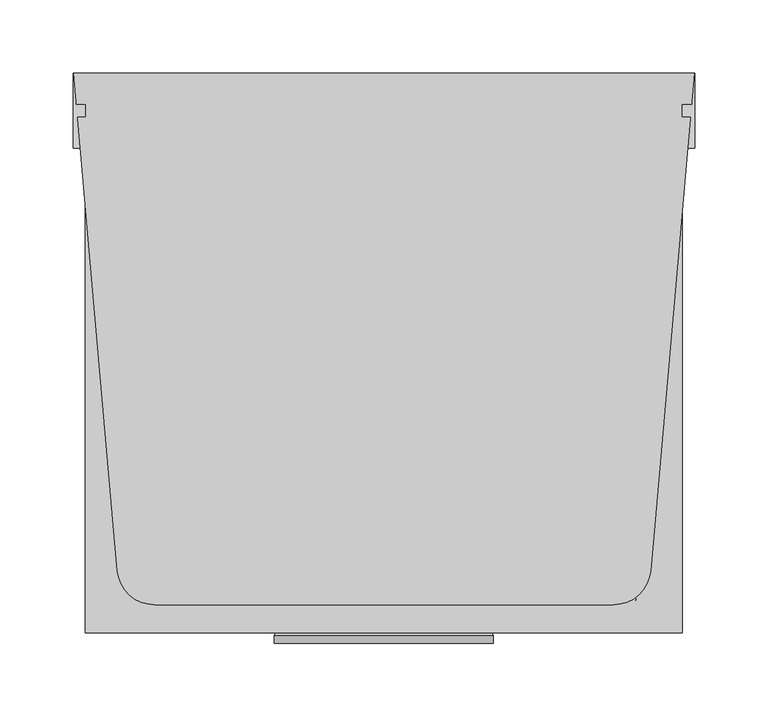
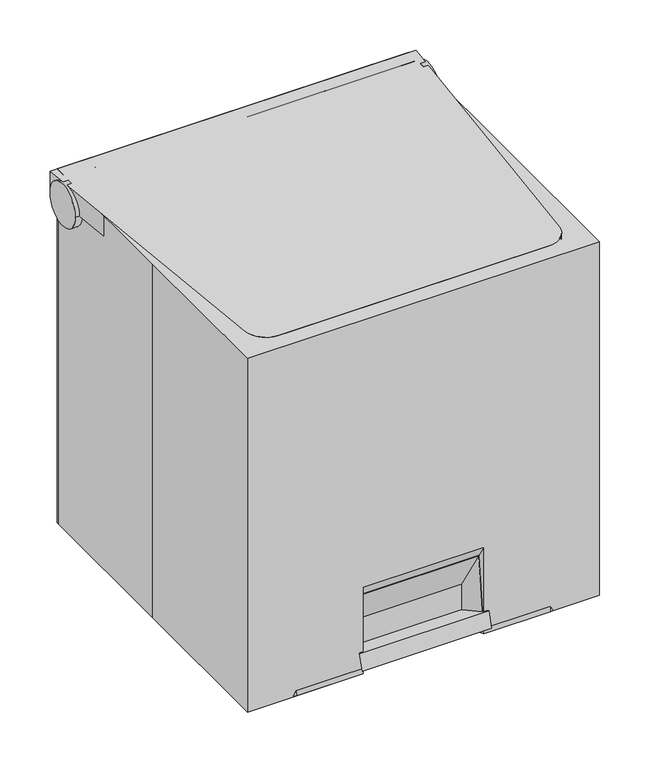
"""IFC4 building model written with IfcOpenShell, lengths in millimetres: proxy geometry, M3073 - Basket, Infectious Waste, Step-On : M0013 - Basket, Infectious Waste, Step-On."""

import ifcopenshell
import ifcopenshell.guid

model = None  # the IFC model being written
_history = None  # IfcOwnerHistory: only IFC2X3 demands one
_inside = {}  # id of a spatial element -> (the spatial element, [elements in it])
_under = {}  # id of a project, library or spatial element -> (it, [spatial elements below it])
_declared = {}  # id of a project -> (the project, [libraries it declares])
_typed = {}  # id of a type object -> (the type object, [elements of that type])
_made_of = {}  # id of a material, layer set ... -> (it, [elements and type objects made of it])


def new_model(schema):
    """Start an empty IFC model of exactly this schema.

    Asked for "IFC4X3", IfcOpenShell would pick the latest addendum, in which some entities
    have other attributes; the version numbers below select the first issue.
    IFC2X3 requires an IfcOwnerHistory on every rooted entity: one is made here for all.
    """
    global model, _history
    if schema == "IFC4X3":
        model = ifcopenshell.file(schema_version=(4, 3, 0, 0))
    else:
        model = ifcopenshell.file(schema=schema)
    _inside.clear()
    _under.clear()
    _declared.clear()
    _typed.clear()
    _made_of.clear()
    _history = None
    if model.schema == "IFC2X3":
        org = make("IfcOrganization", Name="unknown")
        user = make(
            "IfcPersonAndOrganization",
            ThePerson=make("IfcPerson", FamilyName="unknown"),
            TheOrganization=org,
        )
        app = make(
            "IfcApplication",
            ApplicationDeveloper=org,
            Version="unknown",
            ApplicationFullName="unknown",
            ApplicationIdentifier="unknown",
        )
        _history = make(
            "IfcOwnerHistory",
            OwningUser=user,
            OwningApplication=app,
            ChangeAction="ADDED",
            CreationDate=0,
        )
    return model


def make(cls, **values):
    """One entity of the class cls with the attributes given. An attribute that is None is left unset."""
    return model.create_entity(
        cls, **{name: value for name, value in values.items() if value is not None}
    )


def rooted(cls, **values):
    """An entity with a GlobalId (a new one), such as an element, a storey or a relation."""
    return make(cls, GlobalId=ifcopenshell.guid.new(), OwnerHistory=_history, **values)


def si_unit(unit_type, name, prefix=None):
    """IfcSIUnit, for example si_unit("LENGTHUNIT", "METRE", prefix="MILLI")."""
    return make("IfcSIUnit", UnitType=unit_type, Prefix=prefix, Name=name)


def assignment(units):
    """IfcUnitAssignment: the units of a project."""
    return None if units is None else make("IfcUnitAssignment", Units=units)


def point(xyz):
    """IfcCartesianPoint."""
    return None if xyz is None else make("IfcCartesianPoint", Coordinates=xyz)


def direction(xyz):
    """IfcDirection."""
    return None if xyz is None else make("IfcDirection", DirectionRatios=xyz)


def frame(location, z_axis=None, x_axis=None):
    """IfcAxis2Placement3D, a coordinate frame: its origin and axes. An axis left out is left unset."""
    return make(
        "IfcAxis2Placement3D",
        Location=point(location),
        Axis=direction(z_axis),
        RefDirection=direction(x_axis),
    )


def frame_2d(location, x_axis=None):
    """IfcAxis2Placement2D, a coordinate frame in the plane: its origin and x axis."""
    return make(
        "IfcAxis2Placement2D", Location=point(location), RefDirection=direction(x_axis)
    )


def origin():
    """The frame at (0, 0, 0) with its axes left unset."""
    return frame((0.0, 0.0, 0.0))


def place(relative_to, where):
    """IfcLocalPlacement: puts the frame where relative to a parent placement (None: the world)."""
    return make(
        "IfcLocalPlacement", PlacementRelTo=relative_to, RelativePlacement=where
    )


def context(
    kind, dimensions, precision=None, world=None, true_north=None, identifier=None
):
    """IfcGeometricRepresentationContext, for example the 3D "Model" context."""
    return make(
        "IfcGeometricRepresentationContext",
        ContextIdentifier=identifier,
        ContextType=kind,
        CoordinateSpaceDimension=dimensions,
        Precision=precision,
        WorldCoordinateSystem=world,
        TrueNorth=true_north,
    )


def project(units=None, contexts=None):
    """IfcProject with its units and contexts."""
    return rooted(
        "IfcProject",
        Name="project",
        RepresentationContexts=contexts,
        UnitsInContext=assignment(units),
    )


def spatial(cls, under=None, at=None, **own):
    """A site, building, storey or space (cls), placed at a placement, below another one or the project."""
    s = rooted(cls, ObjectPlacement=at, **own)
    if under is not None:
        _under.setdefault(under.id(), (under, []))[1].append(s)
    return s


def polyline(points):
    """IfcPolyline through the points."""
    return make("IfcPolyline", Points=[point(p) for p in points])


def circle_curve(where, radius):
    """IfcCircle in the frame where."""
    return make("IfcCircle", Position=where, Radius=radius)


def ellipse_curve(where, semi_axis1, semi_axis2):
    """IfcEllipse in the frame where."""
    return make(
        "IfcEllipse", Position=where, SemiAxis1=semi_axis1, SemiAxis2=semi_axis2
    )


def trimmed(basis, trim1, trim2, sense, master):
    """IfcTrimmedCurve: the piece of a basis curve between two trims."""
    return make(
        "IfcTrimmedCurve",
        BasisCurve=basis,
        Trim1=trim1,
        Trim2=trim2,
        SenseAgreement=sense,
        MasterRepresentation=master,
    )


def segment(curve, same_sense, transition):
    """IfcCompositeCurveSegment."""
    return make(
        "IfcCompositeCurveSegment",
        Transition=transition,
        SameSense=same_sense,
        ParentCurve=curve,
    )


def composite_curve(segments, self_intersect=None):
    """IfcCompositeCurve: segments joined end to end."""
    return make("IfcCompositeCurve", Segments=segments, SelfIntersect=self_intersect)


def outline(outer, holes=None, kind="AREA"):
    """IfcArbitraryClosedProfileDef: a profile drawn as a closed curve; with holes, ...WithVoids."""
    if holes is None:
        return make("IfcArbitraryClosedProfileDef", ProfileType=kind, OuterCurve=outer)
    return make(
        "IfcArbitraryProfileDefWithVoids",
        ProfileType=kind,
        OuterCurve=outer,
        InnerCurves=holes,
    )


def extrude(swept, where, along, depth):
    """IfcExtrudedAreaSolid: the profile swept, set in the frame where, extruded along a direction by depth."""
    return make(
        "IfcExtrudedAreaSolid",
        SweptArea=swept,
        Position=where,
        ExtrudedDirection=direction(along),
        Depth=depth,
    )


def shape(context_of_items, identifier, shape_type, items):
    """IfcShapeRepresentation: the items that make up one representation, for example the "Body"."""
    return make(
        "IfcShapeRepresentation",
        ContextOfItems=context_of_items,
        RepresentationIdentifier=identifier,
        RepresentationType=shape_type,
        Items=items,
    )


def source(mapping_origin, context_of_items, identifier, shape_type, items):
    """IfcRepresentationMap: a shape defined once, which mapped items show again and again."""
    return make(
        "IfcRepresentationMap",
        MappingOrigin=mapping_origin,
        MappedRepresentation=shape(context_of_items, identifier, shape_type, items),
    )


def transform(
    local_origin,
    x_axis=None,
    y_axis=None,
    z_axis=None,
    scale=None,
    scale2=None,
    scale3=None,
    uniform=True,
):
    """IfcCartesianTransformationOperator3D, or its non-uniform kind. x_axis, y_axis, z_axis: its Axis1, 2, 3."""
    if uniform:
        return make(
            "IfcCartesianTransformationOperator3D",
            Axis1=direction(x_axis),
            Axis2=direction(y_axis),
            LocalOrigin=point(local_origin),
            Scale=scale,
            Axis3=direction(z_axis),
        )
    return make(
        "IfcCartesianTransformationOperator3DnonUniform",
        Axis1=direction(x_axis),
        Axis2=direction(y_axis),
        LocalOrigin=point(local_origin),
        Scale=scale,
        Axis3=direction(z_axis),
        Scale2=scale2,
        Scale3=scale3,
    )


def mapped(mapping_source, mapping_target):
    """IfcMappedItem: shows the shape of a source again, moved by a transform."""
    return make(
        "IfcMappedItem", MappingSource=mapping_source, MappingTarget=mapping_target
    )


def made_of(thing, what):
    """Note that an element or type object is made of a material, layer set ...; save() writes the relation."""
    if what is not None:
        _made_of.setdefault(what.id(), (what, []))[1].append(thing)
    return thing


def element(
    cls,
    number,
    at=None,
    inside=None,
    cuts=None,
    type_object=None,
    material=None,
    context=None,
    identifier="Body",
    shape_type=None,
    held_by="IfcProductDefinitionShape",
    body=None,
    shapes=None,
    **own,
):
    """One element of the class cls, such as IfcWall. Its Tag is "e" and its number.

    at: its placement. inside: the storey or other place that contains it. cuts: it is an
    opening in that element (IfcRelVoidsElement). A single representation is given by context,
    identifier, shape_type and body (its items); several are given by shapes. held_by: the class
    of the entity that holds the representations. save() writes the other relations.
    """
    e = rooted(cls, Tag="e%d" % number, ObjectPlacement=at, **own)
    if body is not None:
        shapes = [shape(context, identifier, shape_type, body)]
    if shapes is not None:
        e.Representation = make(held_by, Representations=shapes)
    if inside is not None:
        _inside.setdefault(inside.id(), (inside, []))[1].append(e)
    if cuts is not None:
        rooted(
            "IfcRelVoidsElement", RelatingBuildingElement=cuts, RelatedOpeningElement=e
        )
    if type_object is not None:
        _typed.setdefault(type_object.id(), (type_object, []))[1].append(e)
    return made_of(e, material)


def aggregate(whole, parts):
    """IfcRelAggregates: a whole, such as a stair, and the parts it consists of."""
    return rooted("IfcRelAggregates", RelatingObject=whole, RelatedObjects=parts)


def save(model, path):
    """Write the relations noted so far, then the file.

    IfcRelAggregates (storeys below a building ...), IfcRelContainedInSpatialStructure (elements
    in a storey), IfcRelDefinesByType, IfcRelAssociatesMaterial and IfcRelDeclares: one each for
    every whole, place, type object, material and project.
    """
    for whole, parts in _under.values():
        aggregate(whole, parts)
    for where, things in _inside.values():
        rooted(
            "IfcRelContainedInSpatialStructure",
            RelatedElements=things,
            RelatingStructure=where,
        )
    for kind, things in _typed.values():
        rooted("IfcRelDefinesByType", RelatedObjects=things, RelatingType=kind)
    for what, things in _made_of.values():
        rooted("IfcRelAssociatesMaterial", RelatedObjects=things, RelatingMaterial=what)
    for by, libraries in _declared.values():
        rooted("IfcRelDeclares", RelatingContext=by, RelatedDefinitions=libraries)
    model.write(path)


def plane_surface(at):
    """IfcPlane: the flat surface through the origin of the frame at, square to its z axis."""
    return make("IfcPlane", Position=at)


def cylinder_surface(at, radius):
    """IfcCylindricalSurface: all points at the distance radius from the z axis of the frame at."""
    return make("IfcCylindricalSurface", Position=at, Radius=radius)


def revolved_surface(curve, axis_point, axis_direction):
    """IfcSurfaceOfRevolution: the curve turned about the line through axis_point along axis_direction."""
    return make(
        "IfcSurfaceOfRevolution",
        SweptCurve=make("IfcArbitraryOpenProfileDef", ProfileType="CURVE", Curve=curve),
        AxisPosition=make("IfcAxis1Placement", Location=point(axis_point), Axis=direction(axis_direction)),
    )


def spline_surface(u_degree, v_degree, points, u_multiplicities, v_multiplicities, u_knots, v_knots, weights=None):
    """IfcBSplineSurfaceWithKnots; with weights, IfcRationalBSplineSurfaceWithKnots. points: one row for each step in u."""
    own = dict(
        UDegree=u_degree,
        VDegree=v_degree,
        ControlPointsList=[[point(p) for p in row] for row in points],
        SurfaceForm="UNSPECIFIED",
        UClosed=False,
        VClosed=False,
        SelfIntersect=False,
        UMultiplicities=u_multiplicities,
        VMultiplicities=v_multiplicities,
        UKnots=u_knots,
        VKnots=v_knots,
        KnotSpec="UNSPECIFIED",
    )
    if weights is None:
        return make("IfcBSplineSurfaceWithKnots", **own)
    return make("IfcRationalBSplineSurfaceWithKnots", WeightsData=weights, **own)


def advanced_brep(points, edges, surfaces, faces):
    """IfcAdvancedBrep: a solid bounded by faces that lie on surfaces and meet in shared edges.

    An edge is (start, end): straight between two places in points (the first is 0);
    or (start, end, curve); or (start, end, curve, False) where it runs against its curve.
    A face is (place in surfaces, loops), or (place, loops, False) where it looks against
    its surface's normal. A loop lists edges by number (the first is 1), with a minus sign
    where the edge is run from its end to its start. The first loop is the outer one.
    """
    corners = [point(p) for p in points]
    vertices = [make("IfcVertexPoint", VertexGeometry=c) for c in corners]
    made = []
    for start, end, *more in edges:
        made.append(
            make(
                "IfcEdgeCurve",
                EdgeStart=vertices[start],
                EdgeEnd=vertices[end],
                EdgeGeometry=more[0] if more else make("IfcPolyline", Points=[corners[start], corners[end]]),
                SameSense=more[1] if len(more) > 1 else True,
            )
        )
    hull = []
    for where, loops, *sense in faces:
        bounds = []
        for j, loop in enumerate(loops):
            ring = [make("IfcOrientedEdge", EdgeElement=made[abs(k) - 1], Orientation=k > 0) for k in loop]
            bounds.append(
                make(
                    "IfcFaceOuterBound" if j == 0 else "IfcFaceBound",
                    Bound=make("IfcEdgeLoop", EdgeList=ring),
                    Orientation=True,
                )
            )
        hull.append(make("IfcAdvancedFace", Bounds=bounds, FaceSurface=surfaces[where], SameSense=sense[0] if sense else True))
    return make("IfcAdvancedBrep", Outer=make("IfcClosedShell", CfsFaces=hull))


def specialty_equipment_3a0a294f(model_context):
    return source(origin(), model_context, "Body", "SolidModel", [
        extrude(outline(composite_curve([segment(trimmed(circle_curve(frame_2d((165.1, 406.4)), 25.4), [point((190.5, 406.4))], [point((139.7, 406.4))], False, "CARTESIAN"), True, "CONTINUOUS"), segment(trimmed(circle_curve(frame_2d((165.1, 406.4)), 25.4), [point((139.7, 406.4))], [point((190.5, 406.4))], False, "CARTESIAN"), True, "CONTINUOUS")], self_intersect=False)), frame((203.2, 0.0, 0.0), z_axis=(1.0, 0.0, 0.0), x_axis=(0.0, 1.0, 0.0)), (0.0, 0.0, 1.0), 8.2243705),
        extrude(outline(composite_curve([segment(trimmed(circle_curve(frame_2d((165.1, 406.4)), 25.4), [point((139.7, 406.4))], [point((190.5, 406.4))], False, "CARTESIAN"), True, "CONTINUOUS"), segment(trimmed(circle_curve(frame_2d((165.1, 406.4)), 25.4), [point((190.5, 406.4))], [point((139.7, 406.4))], False, "CARTESIAN"), True, "CONTINUOUS")], self_intersect=False)), frame((-211.3962544, 0.0, 0.0), z_axis=(1.0, 0.0, 0.0), x_axis=(0.0, 1.0, 0.0)), (0.0, 0.0, 1.0), 8.1962544),
        advanced_brep(
        [(-181.4886497, -148.2637559, 431.8), (-156.1853044, -171.45, 431.8), (156.1853044, -171.45, 431.8), (181.4886497, -148.2637559, 431.8), (211.1266379, 190.5, 431.8), (-211.1266379, 190.5, 431.8), (-181.4886497, -148.2637559, 406.4), (-211.1266379, 190.5, 406.4), (-203.2, 190.5, 406.4), (-203.2, 139.7, 406.4), (203.2, 139.7, 406.4), (203.2, 190.5, 406.4), (211.1266379, 190.5, 406.4), (181.4886497, -148.2637559, 406.4), (156.1853044, -171.45, 406.4), (-156.1853044, -171.45, 406.4), (203.2, 165.1, 431.8), (-203.2, 165.1, 431.8)],
        [
            (0, 1, circle_curve(frame((-156.1853044, -146.05, 431.8), z_axis=(0.0, 0.0, 1.0), x_axis=(1.0, 0.0, 0.0)), 25.4)),
            (1, 2),
            (2, 3, circle_curve(frame((156.1853044, -146.05, 431.8), z_axis=(0.0, 0.0, 1.0), x_axis=(1.0, 0.0, 0.0)), 25.4)),
            (3, 4),
            (4, 5),
            (5, 0),
            (6, 7),
            (7, 8),
            (8, 9),
            (9, 10),
            (10, 11),
            (11, 12),
            (12, 13),
            (13, 14, circle_curve(frame((156.1853044, -146.05, 406.4), z_axis=(0.0, 0.0, -1.0), x_axis=(1.0, 0.0, 0.0)), 25.4)),
            (14, 15),
            (15, 6, circle_curve(frame((-156.1853044, -146.05, 406.4), z_axis=(0.0, 0.0, -1.0), x_axis=(1.0, 0.0, 0.0)), 25.4)),
            (0, 6),
            (15, 1),
            (14, 2),
            (13, 3),
            (12, 4),
            (11, 8),
            (7, 5),
            (10, 16, circle_curve(frame((203.2, 165.1, 406.4), z_axis=(-1.0, 0.0, 0.0), x_axis=(0.0, 1.0, 0.0)), 25.4)),
            (16, 11, circle_curve(frame((203.2, 165.1, 406.4), z_axis=(-1.0, 0.0, 0.0), x_axis=(0.0, 1.0, 0.0)), 25.4)),
            (8, 17, circle_curve(frame((-203.2, 165.1, 406.4), z_axis=(1.0, 0.0, 0.0), x_axis=(0.0, 1.0, 0.0)), 25.4)),
            (17, 9, circle_curve(frame((-203.2, 165.1, 406.4), z_axis=(1.0, 0.0, 0.0), x_axis=(0.0, 1.0, 0.0)), 25.4)),
        ],
        [
            plane_surface(frame((-130.7853044, -146.05, 431.8), z_axis=(0.0, 0.0, 1.0), x_axis=(0.0, 1.0, 0.0))),
            plane_surface(frame((-130.7853044, -146.05, 406.4), z_axis=(0.0, 0.0, -1.0), x_axis=(0.0, -1.0, 0.0))),
            cylinder_surface(frame((-156.1853044, -146.05, 406.4), z_axis=(0.0, 0.0, 1.0), x_axis=(1.0, 0.0, 0.0)), 25.4),
            plane_surface(frame((-156.1853044, -171.45, 431.8), z_axis=(0.0, -1.0, 0.0), x_axis=(0.0, 0.0, -1.0))),
            cylinder_surface(frame((156.1853044, -146.05, 406.4), z_axis=(0.0, 0.0, 1.0), x_axis=(1.0, 0.0, 0.0)), 25.4),
            plane_surface(frame((181.4886497, -148.2637559, 431.8), z_axis=(0.9961946980917455, -0.08715574274765969, 0.0), x_axis=(0.0, 0.0, -1.0))),
            plane_surface(frame((211.1266379, 190.5, 431.8), z_axis=(0.0, 1.0, 0.0), x_axis=(0.0, 0.0, -1.0))),
            plane_surface(frame((-211.1266379, 190.5, 431.8), z_axis=(-0.9961946980917458, -0.08715574274765654, 0.0), x_axis=(0.0, 0.0, -1.0))),
            plane_surface(frame((203.2, 190.5, 406.4), z_axis=(-1.0, 0.0, 0.0), x_axis=(0.0, 0.0, 1.0))),
            plane_surface(frame((-203.2, 190.5, 406.4), z_axis=(1.0, 0.0, 0.0), x_axis=(0.0, 0.0, -1.0))),
            revolved_surface(polyline([(203.2, 190.5, 406.4), (-203.2, 190.5, 406.4)]), (-203.2, 165.1, 406.4), (1.0, 0.0, 0.0)),
        ],
        [
            (0, [[1, 2, 3, 4, 5, 6]]),
            (1, [[7, 8, 9, 10, 11, 12, 13, 14, 15, 16]]),
            (2, [[-1, 17, -16, 18]]),
            (3, [[-2, -18, -15, 19]]),
            (4, [[-3, -19, -14, 20]]),
            (5, [[-4, -20, -13, 21]]),
            (6, [[-5, -21, -12, 22, -8, 23]]),
            (7, [[-6, -23, -7, -17]]),
            (8, [[24, 25, -11]]),
            (9, [[26, 27, -9]]),
            (10, [[-24, -10, -27, -26, -22, -25]]),
        ],
    ),
        advanced_brep(
        [(-171.8953527, -167.3137559, 406.4), (171.8953527, -167.3137559, 406.4), (198.7555759, 139.7, 406.4), (-198.7555759, 139.7, 406.4), (203.2, 190.5, 0.0), (171.8953527, -167.3137559, 0.0), (146.5920074, -190.5, 0.0), (69.85, -190.5, 0.0), (57.15, -167.3137559, 0.0), (-57.15, -167.3137559, 0.0), (-69.85, -190.5, 0.0), (-146.5920074, -190.5, 0.0), (-171.8953527, -167.3137559, 0.0), (-203.2, 190.5, 0.0), (-203.2, 190.5, 406.4), (203.2, 190.5, 406.4), (-66.9435562, -185.1937389, 93.0062024), (66.9435562, -185.1937389, 93.0062024), (57.15, -167.3137559, 50.8), (-57.15, -167.3137559, 50.8)],
        [
            (0, 1),
            (1, 2),
            (2, 3),
            (3, 0),
            (4, 5),
            (5, 6, circle_curve(frame((146.5920074, -165.1, 0.0), z_axis=(0.0, 0.0, -1.0), x_axis=(1.0, 0.0, 0.0)), 25.4)),
            (6, 7),
            (7, 8),
            (8, 9),
            (9, 10),
            (10, 11),
            (11, 12, circle_curve(frame((-146.5920074, -165.1, 0.0), z_axis=(0.0, 0.0, -1.0), x_axis=(1.0, 0.0, 0.0)), 25.4)),
            (12, 13),
            (13, 4),
            (13, 14),
            (14, 15),
            (15, 4),
            (12, 0),
            (3, 14, ellipse_curve(frame((-200.9777879, 165.1, 406.4), z_axis=(0.9961946980917457, 0.08715574274765671, 0.0), x_axis=(0.08715574274765668, -0.9961946980917457, 0.0)), 25.4970239, 25.4)),
            (11, 0),
            (10, 16),
            (16, 17),
            (17, 7),
            (6, 1),
            (5, 1),
            (15, 2, ellipse_curve(frame((200.9777879, 165.1, 406.4), z_axis=(-0.9961946980917454, 0.08715574274765969, 0.0), x_axis=(0.0871557427476588, 0.9961946980917455, 0.0)), 25.4970239, 25.4)),
            (18, 19),
            (19, 9),
            (8, 18),
            (18, 17),
            (16, 19),
        ],
        [
            plane_surface(frame((0.0, 11.5931221, 406.4), z_axis=(0.0, 0.0, 1.0), x_axis=(0.08715574274765671, -0.9961946980917457, 0.0))),
            plane_surface(frame((0.0, -55.771252, 0.0), z_axis=(0.0, 0.0, -1.0), x_axis=(0.08715574274765671, -0.9961946980917457, 0.0))),
            plane_surface(frame((0.0, 190.5, 0.0), z_axis=(0.0, 1.0, 0.0), x_axis=(-1.0, 0.0, 0.0))),
            plane_surface(frame((-187.5476764, 11.5931221, 0.0), z_axis=(-0.9961946980917457, -0.08715574274765671, 0.0), x_axis=(0.08715574274765671, -0.9961946980917457, 0.0))),
            spline_surface(2, 1, [[(-171.8953527, -167.3137559, 0.0), (-171.8953527, -167.3137559, 406.4)], [(-169.86681913406716, -190.49999996929208, 0.0), (-171.8953527, -167.3137559, 406.4)], [(-146.5920074, -190.5, 0.0), (-171.8953527, -167.3137559, 406.4)]], [3, 3], [2, 2], [0.0, 1.0], [0.0, 1.0], weights=[[1.0, 1.0], [0.7372773377124887, 0.7372773377124887], [1.0, 1.0]]),
            plane_surface(frame((0.0, -190.5, 0.0), z_axis=(0.0, -0.9983764533733115, 0.05696013825236224), x_axis=(1.0, 0.0, 0.0))),
            spline_surface(2, 1, [[(146.5920074, -190.5, 0.0), (171.8953527, -167.3137559, 406.4)], [(169.86681918616762, -190.5000000261497, 0.0), (171.8953527, -167.3137559, 406.4)], [(171.8953527, -167.3137559, 0.0), (171.8953527, -167.3137559, 406.4)]], [3, 3], [2, 2], [0.0, 1.0], [0.0, 1.0], weights=[[1.0, 1.0], [0.7372773368872948, 0.7372773368872948], [1.0, 1.0]]),
            plane_surface(frame((187.5476764, 11.5931221, 0.0), z_axis=(0.9961946980917454, -0.08715574274765969, 0.0), x_axis=(0.08715574274765969, 0.9961946980917454, 0.0))),
            plane_surface(frame((0.0, -167.3137559, 25.4), z_axis=(0.0, -1.0, 0.0), x_axis=(-1.0, 0.0, 0.0))),
            plane_surface(frame((0.0, -190.5, 105.5317808), z_axis=(0.0, -0.920783074067558, -0.39007503189860543), x_axis=(1.0, 0.0, 0.0))),
            plane_surface(frame((-69.85, -190.5, 52.7658904), z_axis=(0.8770521055181142, -0.48039525830949104, 0.0), x_axis=(0.0, 0.0, 1.0))),
            plane_surface(frame((69.85, -190.5, 52.7658904), z_axis=(-0.8770521055181134, -0.48039525830949253, 0.0), x_axis=(0.0, 0.0, -1.0))),
            revolved_surface(polyline([(203.2, 190.5, 406.4), (-203.2, 190.5, 406.4)]), (-203.2, 165.1, 406.4), (1.0, 0.0, 0.0)),
        ],
        [
            (0, [[1, 2, 3, 4]]),
            (1, [[5, 6, 7, 8, 9, 10, 11, 12, 13, 14]]),
            (2, [[-14, 15, 16, 17]]),
            (3, [[-13, 18, -4, 19, -15]]),
            (4, [[-12, 20, -18]]),
            (5, [[-1, -20, -11, 21, 22, 23, -7, 24]]),
            (6, [[-6, 25, -24]]),
            (7, [[-5, -17, 26, -2, -25]]),
            (8, [[27, 28, -9, 29]]),
            (9, [[-27, 30, -22, 31]]),
            (10, [[-28, -31, -21, -10]]),
            (11, [[-29, -8, -23, -30]]),
            (12, [[-3, -26, -16, -19]]),
        ],
    ),
        extrude(outline(polyline([(4.6906993, 0.0), (-12.7, -31.75), (-127.0, -31.75), (-144.3906993, 0.0), (4.6906993, 0.0)])), frame((-69.85, -197.7247404, 9.1232954), z_axis=(0.0, 0.2873478855663447, 0.9578262852211517), x_axis=(-1.0, 0.0, 0.0)), (0.0, 0.0, 1.0), 19.05),
        advanced_brep(
        [(-203.2, 0.0, 431.8), (-203.2, -190.5, 431.8), (203.2, -190.5, 431.8), (203.2, 165.1, 431.8), (203.2, 190.5, 431.8), (-203.2, 190.5, 431.8), (-203.2, 165.1, 431.8), (-203.2, 190.5, 0.0), (203.2, 190.5, 0.0), (203.2, -190.5, 0.0), (69.85, -190.5, 0.0), (57.15, -167.3137559, 0.0), (-57.15, -167.3137559, 0.0), (-69.85, -190.5, 0.0), (-203.2, -190.5, 0.0), (-203.2, 0.0, 0.0), (-203.2, 190.5, 406.4), (-203.2, 139.7, 406.4), (-69.85, -190.5, 105.5317808), (69.85, -190.5, 105.5317808), (203.2, 190.5, 406.4), (203.2, 139.7, 406.4), (57.15, -167.3137559, 50.8), (-57.15, -167.3137559, 50.8)],
        [
            (0, 1),
            (1, 2),
            (2, 3),
            (3, 4),
            (4, 5),
            (5, 6),
            (6, 0),
            (7, 8),
            (8, 9),
            (9, 10),
            (10, 11),
            (11, 12),
            (12, 13),
            (13, 14),
            (14, 15),
            (15, 7),
            (5, 16),
            (16, 6, circle_curve(frame((-203.2, 165.1, 406.4), z_axis=(1.0, 0.0, 0.0), x_axis=(0.0, 1.0, 0.0)), 25.4)),
            (15, 0),
            (6, 17, circle_curve(frame((-203.2, 165.1, 406.4), z_axis=(1.0, 0.0, 0.0), x_axis=(0.0, 1.0, 0.0)), 25.4)),
            (17, 16, circle_curve(frame((-203.2, 165.1, 406.4), z_axis=(1.0, 0.0, 0.0), x_axis=(0.0, 1.0, 0.0)), 25.4)),
            (16, 7),
            (14, 1),
            (13, 18),
            (18, 19),
            (19, 10),
            (9, 2),
            (3, 20, circle_curve(frame((203.2, 165.1, 406.4), z_axis=(-1.0, 0.0, 0.0), x_axis=(0.0, 1.0, 0.0)), 25.4)),
            (20, 4),
            (8, 20),
            (20, 21, circle_curve(frame((203.2, 165.1, 406.4), z_axis=(-1.0, 0.0, 0.0), x_axis=(0.0, 1.0, 0.0)), 25.4)),
            (21, 3, circle_curve(frame((203.2, 165.1, 406.4), z_axis=(-1.0, 0.0, 0.0), x_axis=(0.0, 1.0, 0.0)), 25.4)),
            (22, 23),
            (23, 12),
            (11, 22),
            (22, 19),
            (18, 23),
            (20, 16),
            (17, 21),
        ],
        [
            plane_surface(frame((-203.2, 0.0, 431.8), z_axis=(0.0, 0.0, 1.0), x_axis=(0.0, -1.0, 0.0))),
            plane_surface(frame((-203.2, 0.0, 0.0), z_axis=(0.0, 0.0, -1.0), x_axis=(0.0, 1.0, 0.0))),
            plane_surface(frame((-203.2, 190.5, 431.8), z_axis=(-1.0, 0.0, 0.0), x_axis=(0.0, 0.0, -1.0))),
            plane_surface(frame((-203.2, 0.0, 431.8), z_axis=(-1.0, 0.0, 0.0), x_axis=(0.0, 0.0, -1.0))),
            plane_surface(frame((-203.2, -190.5, 431.8), z_axis=(0.0, -1.0, 0.0), x_axis=(0.0, 0.0, -1.0))),
            plane_surface(frame((203.2, -190.5, 431.8), z_axis=(1.0, 0.0, 0.0), x_axis=(0.0, 0.0, -1.0))),
            plane_surface(frame((203.2, 190.5, 431.8), z_axis=(0.0, 1.0, 0.0), x_axis=(0.0, 0.0, -1.0))),
            plane_surface(frame((0.0, -167.3137559, 25.4), z_axis=(0.0, -1.0, 0.0), x_axis=(-1.0, 0.0, 0.0))),
            plane_surface(frame((0.0, -190.5, 105.5317808), z_axis=(0.0, -0.920783074067558, -0.39007503189860543), x_axis=(1.0, 0.0, 0.0))),
            plane_surface(frame((-69.85, -190.5, 52.7658904), z_axis=(0.8770521055181142, -0.48039525830949104, 0.0), x_axis=(0.0, 0.0, 1.0))),
            plane_surface(frame((69.85, -190.5, 52.7658904), z_axis=(-0.8770521055181134, -0.48039525830949253, 0.0), x_axis=(0.0, 0.0, -1.0))),
            revolved_surface(polyline([(203.2, 190.5, 406.4), (-203.2, 190.5, 406.4)]), (-203.2, 165.1, 406.4), (1.0, 0.0, 0.0)),
        ],
        [
            (0, [[1, 2, 3, 4, 5, 6, 7]]),
            (1, [[8, 9, 10, 11, 12, 13, 14, 15, 16]]),
            (2, [[-6, 17, 18]]),
            (2, [[-16, 19, -7, 20, 21, 22]]),
            (3, [[-1, -19, -15, 23]]),
            (4, [[-2, -23, -14, 24, 25, 26, -10, 27]]),
            (5, [[-4, 28, 29]]),
            (5, [[-9, 30, 31, 32, -3, -27]]),
            (6, [[-5, -29, -30, -8, -22, -17]]),
            (7, [[33, 34, -12, 35]]),
            (8, [[-33, 36, -25, 37]]),
            (9, [[-34, -37, -24, -13]]),
            (10, [[-35, -11, -26, -36]]),
            (11, [[38, -21, 39, -31]]),
            (11, [[-38, -28, -32, -39, -20, -18]]),
        ],
    ),
    ])


if __name__ == "__main__":
    model = new_model("IFC4")
    model_context = context("Model", 3, world=origin())
    ifc_project = project(units=[si_unit("LENGTHUNIT", "METRE", prefix="MILLI")], contexts=[model_context])
    site = spatial("IfcSite", under=ifc_project)
    building = spatial("IfcBuilding", under=site)
    placement = place(None, origin())
    specialty_equipment_shape = specialty_equipment_3a0a294f(model_context)
    element("IfcBuildingElementProxy", 1, Name="M3073 - Basket, Infectious Waste, Step-On : M0013 - Basket, Infectious Waste, Step-On", ObjectType="M3073 - Basket, Infectious Waste, Step-On : M0013 - Basket, Infectious Waste, Step-On", at=placement, inside=building, context=model_context, shape_type="MappedRepresentation", body=[
        mapped(specialty_equipment_shape, transform((0.0, 0.0, 0.0), x_axis=(1.0, 0.0, 0.0), y_axis=(0.0, 1.0, 0.0), z_axis=(0.0, 0.0, 1.0))),
    ])
    save(model, "model.ifc")

# Revit data of these elements
# Project information
#   Room Abbreviation = "ORNS1"
#   Room Description = "Operating Room, Neurology (ORNS1)"
#   Sheets - Total = "7"
#   Project Issue Date = "Issue Date"
#   Project Status = "Project Status"
#   Client Name = "Owner"
#   Project Address = "Enter address here"
#   Project Name = "Project Name"
#   Project Number = "Project Number"
#   Publication Date = "30-Jan-15"
# Type "M3073 - Basket, Infectious Waste, Step-On : M0013 - Basket, Infectious Waste, Step-On"
#   Watts2 = "0"
#   Watts1 = "0"
#   Unit_Issue = "EA"
#   UTIL_6_Misc = "-"
#   UTIL_5_NonMedGas = "-"
#   UTIL_4_MiscGas = "-"
#   UTIL_3_MedGas = "-"
#   UTIL_2_Elec = "-"
#   UTIL_1_WaterDrain = "-"
#   Nomenclature = "Container, Biohazard Waste, Step-on, Fire Safe"
#   NSN = ""
#   Location [instance default] = ""
#   JSN = "M3073"
#   Fund_Source_VA = "-"
#   Fund_Source_Navy = "-"
#   Fund_Source_Army = "-"
#   Fund_Source_AF = "-"
#   ELEC_Volts2 = "0"
#   ELEC_Volts1 = "0"
#   ELEC_Phase2 = "0"
#   ELEC_Phase1 = "0"
#   ELEC_HertzSwitch = "0"
#   ELEC_HertzDependent = "0"
#   ELEC_Hertz = "0"
#   ELEC_Amps2 = "0"
#   ELEC_Amps1 = "0"
#   DetailDescription = ""
#   CAT_VA = "C"
#   CAT_Navy = "C"
#   CAT_IHS = "-"
#   CAT_Army = "C"
#   CAT_AF = "C"
#   BTUperhour = "0"
#   Weight_IP = 12
#   DIM_Width_IP = 1' - 4"
#   DIM_Height_IP = 1' - 5"
#   DIM_Depth_IP = 1' - 3"
#   Assembly Code = ""
# Element 1 (IfcBuildingElementProxy, "M3073 - Basket, Infectious Waste, Step-On : M0013 - Basket, Infectious Waste, Step-On")
#   Materials on its faces: "EquipSpace"
# Materials
#   "EquipSpace": class "Unassigned", colour RGB 221 217 195, transparency 0.5
